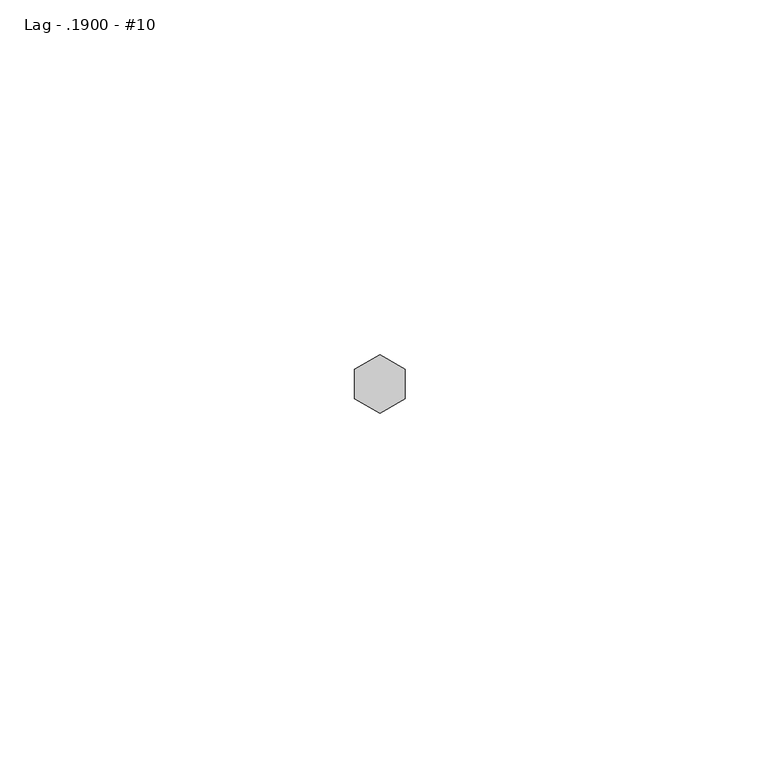
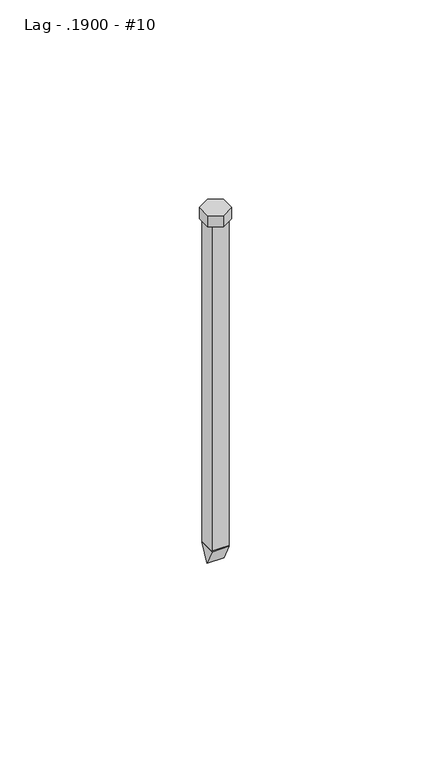
"""IFC4 building model written with IfcOpenShell, lengths in millimetres: fastener geometry, 060523 - W_P_C - Fastenings - Generic - SQUARE : Lag - .1900 - #10."""

from ifc_helpers import new_model, si_unit, frame, origin, origin_with_axes, place, context, project, spatial, polyline, outline, extrude, source, transform, mapped, element, save


def lag_1900_10_e19edac8(model_context):
    return source(origin(), model_context, "Body", "SweptSolid", [
        extrude(outline(polyline([(0.0, -106.6601562), (-2.5300781, -101.6), (2.5300781, -101.6), (0.0, -106.6601562)])), frame((-2.5300781, 0.0, 0.0), z_axis=(1.0, 0.0, 0.0), x_axis=(0.0, 1.0, 0.0)), (0.0, 0.0, 1.0), 5.0601563),
        extrude(outline(polyline([(-3.571875, 2.062223), (0.0, 4.124446), (3.571875, 2.062223), (3.571875, -2.062223), (0.0, -4.124446), (-3.571875, -2.062223), (-3.571875, 2.062223)])), origin_with_axes(), (0.0, 0.0, 1.0), 3.571875),
        extrude(outline(polyline([(-2.5300781, 2.5300781), (2.5300781, 2.5300781), (2.5300781, -2.5300781), (-2.5300781, -2.5300781), (-2.5300781, 2.5300781)])), frame((0.0, 0.0, -101.6), z_axis=(0.0, 0.0, 1.0), x_axis=(1.0, 0.0, 0.0)), (0.0, 0.0, 1.0), 101.6),
    ])


if __name__ == "__main__":
    model = new_model("IFC4")
    model_context = context("Model", 3, world=origin())
    ifc_project = project(units=[si_unit("LENGTHUNIT", "METRE", prefix="MILLI")], contexts=[model_context])
    site = spatial("IfcSite", under=ifc_project)
    building = spatial("IfcBuilding", under=site)
    placement = place(None, origin())
    lag_1900_10_shape = lag_1900_10_e19edac8(model_context)
    element("IfcFastener", 1, ObjectType="060523 - W_P_C - Fastenings - Generic - SQUARE : Lag - .1900 - #10", at=placement, inside=building, context=model_context, shape_type="MappedRepresentation", body=[
        mapped(lag_1900_10_shape, transform((0.0, 0.0, 0.0), x_axis=(1.0, 0.0, 0.0), y_axis=(0.0, 1.0, 0.0), z_axis=(0.0, 0.0, 1.0))),
    ])
    save(model, "model.ifc")

# Revit data of these elements
# Type "060523 - W_P_C - Fastenings - Generic - SQUARE : Lag - .1900 - #10"
#   Washer_Thickness = 0' - 0 3/64"
#   Washer Radius = 0' - 0.24023"
#   Washer Offset - Head = 0' - 0"
#   Washer Offset = 0' - 0"
#   Thickness_of_Substrate [instance default] = 0' - 1"
#   Side = 0' - 0.1626"
#   Radius = 0' - 0.09961"
#   Length [instance default] = 0' - 4"
#   Head Size = 0' - 0 9/32"
#   Head Radius = 0' - 0 9/64"
#   Head Height = 0' - 0 9/64"
#   Double Diameter = 0' - 0 51/128"
#   Diameter = 0' - 0 51/256"
#   Default Elevation = 4' - 0"
#   Washer_Nut_Visibility = no
#   Washer_Head_Visibility = no
#   Round_Head_Visibility = no
#   Point Visibility = yes
#   Nut_Visibility = no
#   Hex_Head_Visiblilty = yes
#   Washer Material = none
#   Bolt Material (Size) = AT SILL - FASTENER AT 24" O.C.
# Element 1 (IfcFastener, "060523 - W_P_C - Fastenings - Generic - SQUARE : Lag - .1900 - #10")
#   Materials on its faces: "AT SILL - FASTENER AT 24\" O.C."
# Materials
#   "AT SILL - FASTENER AT 24\" O.C.": class "Generic", colour RGB 120 120 120, transparency 0, Cost = 0
